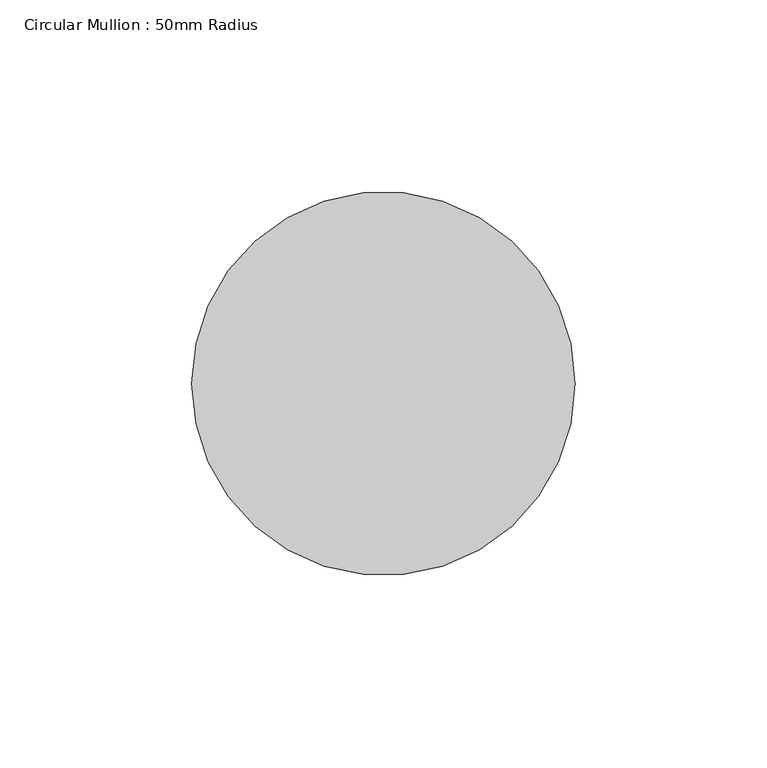
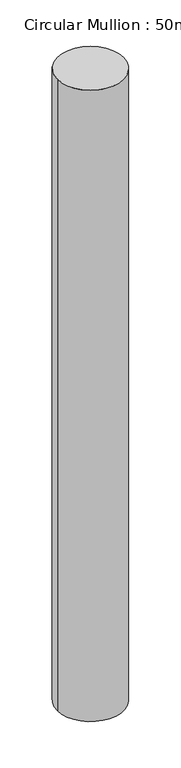
"""IFC4 building model written with IfcOpenShell, lengths in millimetres: member geometry, Circular Mullion : 50mm Radius."""

from ifc_helpers import new_model, si_unit, point, frame, origin, origin_2d, place, context, project, spatial, circle_curve, trimmed, segment, composite_curve, outline, extrude, source, transform, mapped, element, save


def circular_mullion_50mm_radius_090f1352(model_context):
    return source(origin(), model_context, "Body", "SweptSolid", [
        extrude(outline(composite_curve([segment(trimmed(circle_curve(origin_2d(), 50.0), [point((50.0, 0.0))], [point((-50.0, 0.0))], False, "CARTESIAN"), True, "CONTINUOUS"), segment(trimmed(circle_curve(origin_2d(), 50.0), [point((-50.0, 0.0))], [point((50.0, 0.0))], False, "CARTESIAN"), True, "CONTINUOUS")], self_intersect=False)), frame((0.0, 0.0, -1004.8763843), z_axis=(0.0, 0.0, 1.0), x_axis=(1.0, 0.0, 0.0)), (0.0, 0.0, 1.0), 1004.8763843),
    ])


if __name__ == "__main__":
    model = new_model("IFC4")
    model_context = context("Model", 3, world=origin())
    ifc_project = project(units=[si_unit("LENGTHUNIT", "METRE", prefix="MILLI")], contexts=[model_context])
    site = spatial("IfcSite", under=ifc_project)
    building = spatial("IfcBuilding", under=site)
    placement = place(None, origin())
    circular_mullion_50mm_radius_shape = circular_mullion_50mm_radius_090f1352(model_context)
    element("IfcMember", 1, ObjectType="Circular Mullion : 50mm Radius", at=placement, inside=building, context=model_context, shape_type="MappedRepresentation", body=[
        mapped(circular_mullion_50mm_radius_shape, transform((0.0, 0.0, 0.0), x_axis=(1.0, 0.0, 0.0), y_axis=(0.0, 1.0, 0.0), z_axis=(0.0, 0.0, 1.0))),
    ])
    save(model, "model.ifc")

# Revit data of these elements
# Type "Circular Mullion : 50mm Radius"
#   built-in parameter 1007350 = 0.164042 (stored number, unit not read)
# Element 1 (IfcMember, "Circular Mullion : 50mm Radius")
#   Materials on its faces: "Aluminium"
# Materials
#   "Aluminium": class "Metal", colour RGB 247 247 247, transparency 0, Description = "Aluminium 6061", Cost = 0
